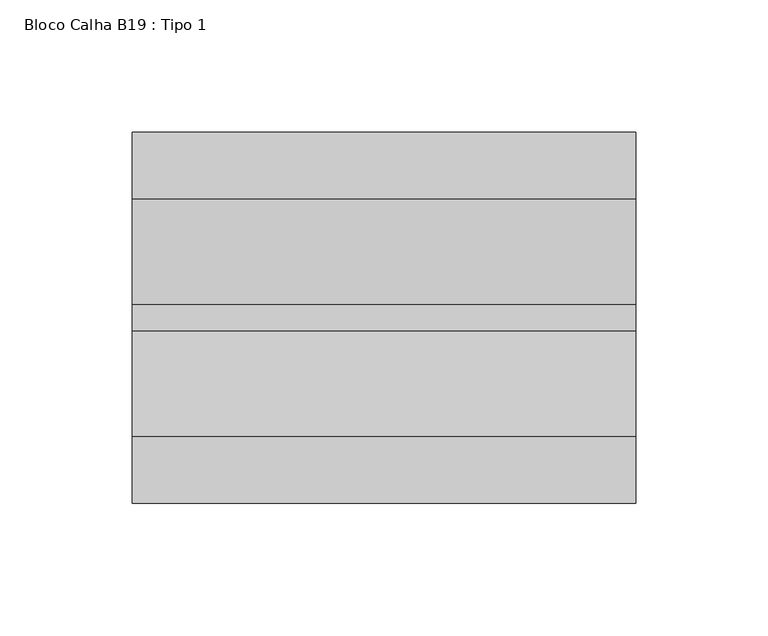
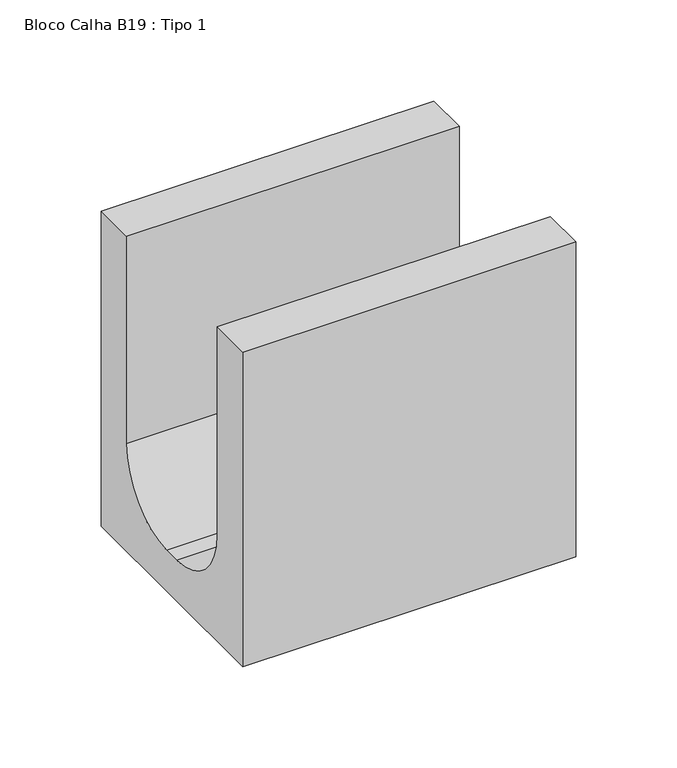
"""IFC4 building model written with IfcOpenShell, lengths in millimetres: proxy geometry, Bloco Calha B19 : Tipo 1."""

from ifc_helpers import new_model, si_unit, point, frame, frame_2d, origin, place, context, project, spatial, polyline, circle_curve, trimmed, segment, composite_curve, outline, extrude, source, transform, mapped, element, save


def bloco_calha_b19_tipo_1_82c6b02f(model_context):
    return source(origin(), model_context, "Body", "SweptSolid", [
        extrude(outline(composite_curve([segment(polyline([(140.0, 0.0), (0.0, 0.0), (0.0, 190.0), (25.0, 190.0), (25.0, 65.0)]), True, "CONTINUOUS"), segment(trimmed(circle_curve(frame_2d((65.0, 65.0)), 40.0), [point((25.0, 65.0))], [point((65.0, 25.0))], True, "CARTESIAN"), True, "CONTINUOUS"), segment(polyline([(65.0, 25.0), (75.0, 25.0)]), True, "CONTINUOUS"), segment(trimmed(circle_curve(frame_2d((75.0, 65.0)), 40.0), [point((75.0, 25.0))], [point((115.0, 65.0))], True, "CARTESIAN"), True, "CONTINUOUS"), segment(polyline([(115.0, 65.0), (115.0, 190.0), (140.0, 190.0), (140.0, 0.0)]), True, "CONTINUOUS")], self_intersect=False)), frame((0.0, 0.0, 0.0), z_axis=(1.0, 0.0, 0.0), x_axis=(0.0, 1.0, 0.0)), (0.0, 0.0, 1.0), 190.0),
    ])


if __name__ == "__main__":
    model = new_model("IFC4")
    model_context = context("Model", 3, world=origin())
    ifc_project = project(units=[si_unit("LENGTHUNIT", "METRE", prefix="MILLI")], contexts=[model_context])
    site = spatial("IfcSite", under=ifc_project)
    building = spatial("IfcBuilding", under=site)
    placement = place(None, origin())
    bloco_calha_b19_tipo_1_shape = bloco_calha_b19_tipo_1_82c6b02f(model_context)
    element("IfcBuildingElementProxy", 1, Name="Bloco Calha B19 : Tipo 1", ObjectType="Bloco Calha B19 : Tipo 1", at=placement, inside=building, context=model_context, shape_type="MappedRepresentation", body=[
        mapped(bloco_calha_b19_tipo_1_shape, transform((0.0, 0.0, 0.0), x_axis=(1.0, 0.0, 0.0), y_axis=(0.0, 1.0, 0.0), z_axis=(0.0, 0.0, 1.0))),
    ])
    save(model, "model.ifc")

# Revit data of these elements
# Type "Bloco Calha B19 : Tipo 1"
#   SINAPI = ""
#   Assembly Code = ""
